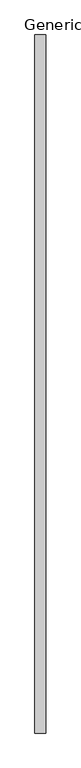
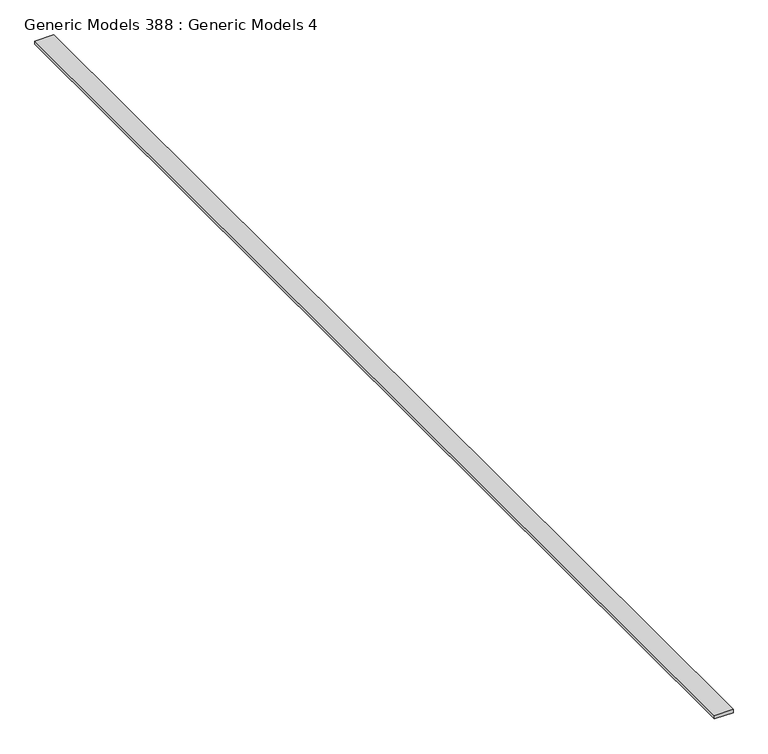
"""IFC4 building model written with IfcOpenShell, lengths in millimetres: proxy geometry, Generic Models 388 : Generic Models 4."""

from ifc_helpers import new_model, si_unit, frame, origin, place, context, project, spatial, polyline, outline, extrude, source, transform, mapped, element, save


def generic_models_388_generic_models_4_e25cc164(model_context):
    return source(origin(), model_context, "Body", "SweptSolid", [
        extrude(outline(polyline([(-6356.5236296, -6864.9230338), (-6458.1236296, -6864.9230338), (-6458.1236296, -464.1230338), (-6356.5236296, -464.1230338), (-6356.5236296, -6864.9230338)])), frame((0.0, 0.0, 127253.8087534), z_axis=(0.0, 0.0, 1.0), x_axis=(1.0, 0.0, 0.0)), (0.0, 0.0, 1.0), 18.9872466),
    ])


if __name__ == "__main__":
    model = new_model("IFC4")
    model_context = context("Model", 3, world=origin())
    ifc_project = project(units=[si_unit("LENGTHUNIT", "METRE", prefix="MILLI")], contexts=[model_context])
    site = spatial("IfcSite", under=ifc_project)
    building = spatial("IfcBuilding", under=site)
    placement = place(None, origin())
    generic_models_388_generic_models_4_shape = generic_models_388_generic_models_4_e25cc164(model_context)
    element("IfcBuildingElementProxy", 1, Name="Generic Models 388 : Generic Models 4", ObjectType="Generic Models 388 : Generic Models 4", at=placement, inside=building, context=model_context, shape_type="MappedRepresentation", body=[
        mapped(generic_models_388_generic_models_4_shape, transform((0.0, 0.0, 0.0), x_axis=(1.0, 0.0, 0.0), y_axis=(0.0, 1.0, 0.0), z_axis=(0.0, 0.0, 1.0))),
    ])
    save(model, "model.ifc")

# Revit data of these elements
# Element 1 (IfcBuildingElementProxy, "Generic Models 388 : Generic Models 4")
#   Materials on its faces: "_HARDWOOD VENEER PLYWOOD (GRADE B, OR BETTER) - MATCH SOLID TRIM SPECIES"
# Materials
#   "_HARDWOOD VENEER PLYWOOD (GRADE B, OR BETTER) - MATCH SOLID TRIM SPECIES": class "Generic", colour RGB 177 130 114, transparency 0, Cost = 0
